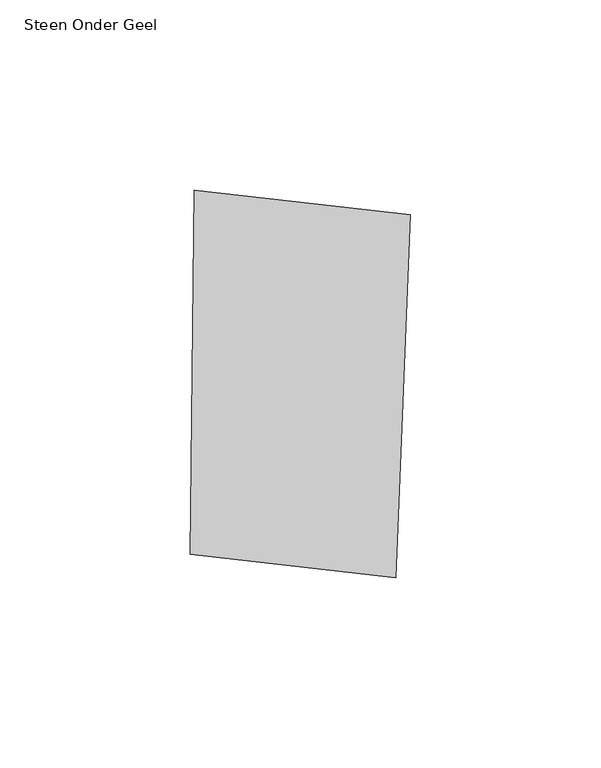
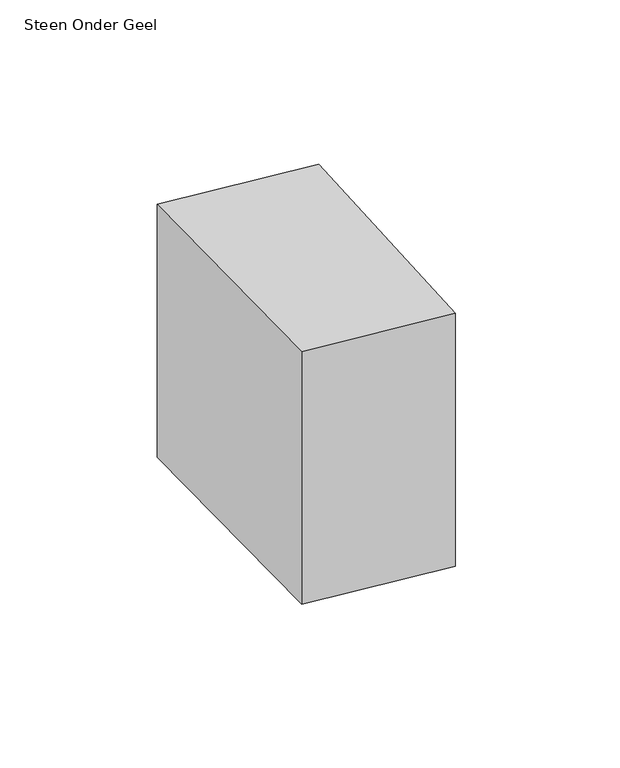
"""IFC4 building model written with IfcOpenShell, lengths in millimetres: proxy geometry, 00_GMA_steen_versie_4 : Steen Onder Geel."""

from ifc_helpers import new_model, si_unit, origin, origin_with_axes, place, context, project, spatial, polyline, outline, extrude, source, transform, mapped, element, save


def steen_onder_geel_e0ac57b3(model_context):
    return source(origin(), model_context, "Body", "SweptSolid", [
        extrude(outline(polyline([(102.3981146, 114.258564), (98.5713319, 19.0678558), (44.610771, 25.1983788), (45.6779233, 120.7134593), (102.3981146, 114.258564)])), origin_with_axes(), (0.0, 0.0, 1.0), 100.0),
    ])


if __name__ == "__main__":
    model = new_model("IFC4")
    model_context = context("Model", 3, world=origin())
    ifc_project = project(units=[si_unit("LENGTHUNIT", "METRE", prefix="MILLI")], contexts=[model_context])
    site = spatial("IfcSite", under=ifc_project)
    building = spatial("IfcBuilding", under=site)
    placement = place(None, origin())
    steen_onder_geel_shape = steen_onder_geel_e0ac57b3(model_context)
    element("IfcBuildingElementProxy", 1, Name="00_GMA_steen_versie_4 : Steen Onder Geel", ObjectType="00_GMA_steen_versie_4 : Steen Onder Geel", at=placement, inside=building, context=model_context, shape_type="MappedRepresentation", body=[
        mapped(steen_onder_geel_shape, transform((0.0, 0.0, 0.0), x_axis=(1.0, 0.0, 0.0), y_axis=(0.0, 1.0, 0.0), z_axis=(0.0, 0.0, 1.0))),
    ])
    save(model, "model.ifc")

# Revit data of these elements
# Type "00_GMA_steen_versie_4 : Steen Onder Geel"
#   StootVoegHalfBoven [instance default] = 5 mm
#   StootVoegHalf [instance default] = 5 mm
#   StootVoegBreedteOnder = 10 mm
#   StootVoegBreedteBoven = 10 mm
#   Steendikte = 100 mm
#   LintVoegOnderHalf = 0 mm
#   LintVoegOnder = 0 mm
#   LintVoegBovenHalf = 5 mm
#   LintVoegBoven = 10 mm
#   materiaal = 21_steen_geel
#   MateriaalVoeg = none
#   Default Elevation = 0
# Element 1 (IfcBuildingElementProxy, "00_GMA_steen_versie_4 : Steen Onder Geel")
#   Materials on its faces: "21_steen_geel"
# Materials
#   "21_steen_geel": class "Unassigned", colour RGB 202 202 0, transparency 0, Cost = 0
